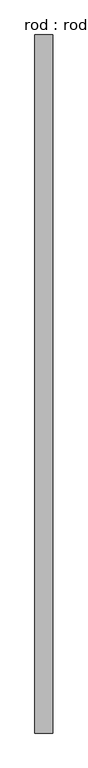
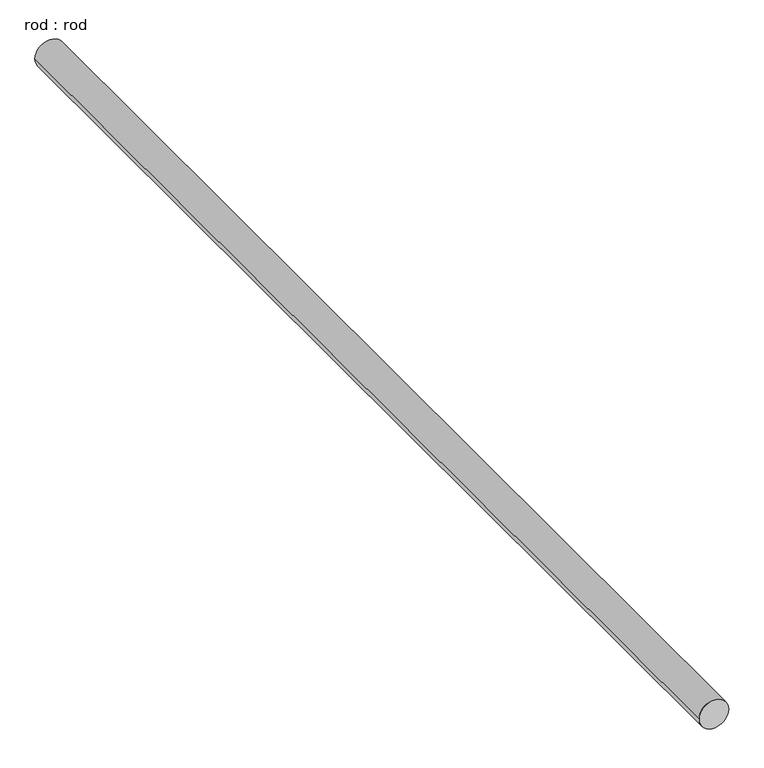
"""IFC4 building model written with IfcOpenShell, lengths in millimetres: proxy geometry, rod : rod."""

from ifc_helpers import new_model, si_unit, point, frame, frame_2d, origin, place, context, project, spatial, circle_curve, trimmed, segment, composite_curve, outline, extrude, source, transform, mapped, element, save


def rod_rod_c199643e(model_context):
    return source(origin(), model_context, "Body", "SweptSolid", [
        extrude(outline(composite_curve([segment(trimmed(circle_curve(frame_2d((0.0108462, 0.0)), 200.0), [point((0.0108462, 200.0))], [point((0.0108462, -200.0))], False, "CARTESIAN"), True, "CONTINUOUS"), segment(trimmed(circle_curve(frame_2d((0.0108462, 0.0)), 200.0), [point((0.0108462, -200.0))], [point((0.0108462, 200.0))], False, "CARTESIAN"), True, "CONTINUOUS")], self_intersect=False)), frame((0.0, -3661.7356704, 0.0), z_axis=(0.0, 1.0, 0.0), x_axis=(0.0, 0.0, 1.0)), (0.0, 0.0, 1.0), 15508.9285714),
    ])


if __name__ == "__main__":
    model = new_model("IFC4")
    model_context = context("Model", 3, world=origin())
    ifc_project = project(units=[si_unit("LENGTHUNIT", "METRE", prefix="MILLI")], contexts=[model_context])
    site = spatial("IfcSite", under=ifc_project)
    building = spatial("IfcBuilding", under=site)
    placement = place(None, origin())
    rod_rod_shape = rod_rod_c199643e(model_context)
    element("IfcBuildingElementProxy", 1, Name="rod : rod", ObjectType="rod : rod", at=placement, inside=building, context=model_context, shape_type="MappedRepresentation", body=[
        mapped(rod_rod_shape, transform((0.0, 0.0, 0.0), x_axis=(1.0, 0.0, 0.0), y_axis=(0.0, 1.0, 0.0), z_axis=(0.0, 0.0, 1.0))),
    ])
    save(model, "model.ifc")

# Revit data of these elements
# Type "rod : rod"
#   Default Elevation = 0
